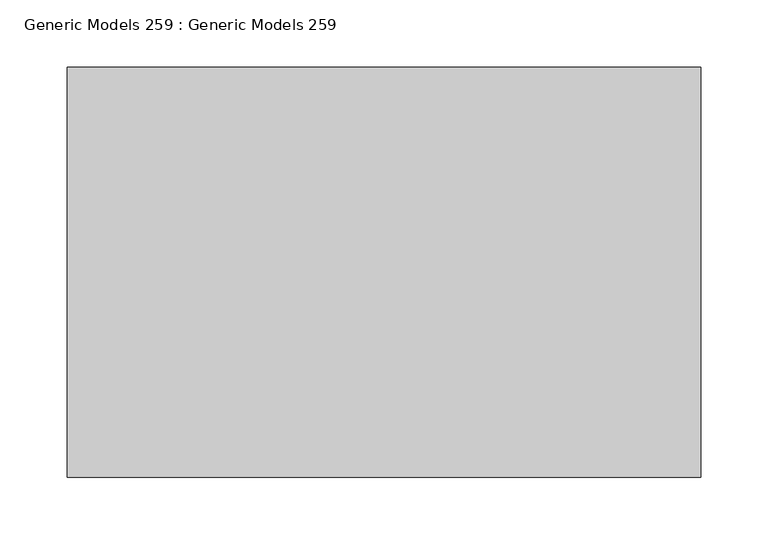
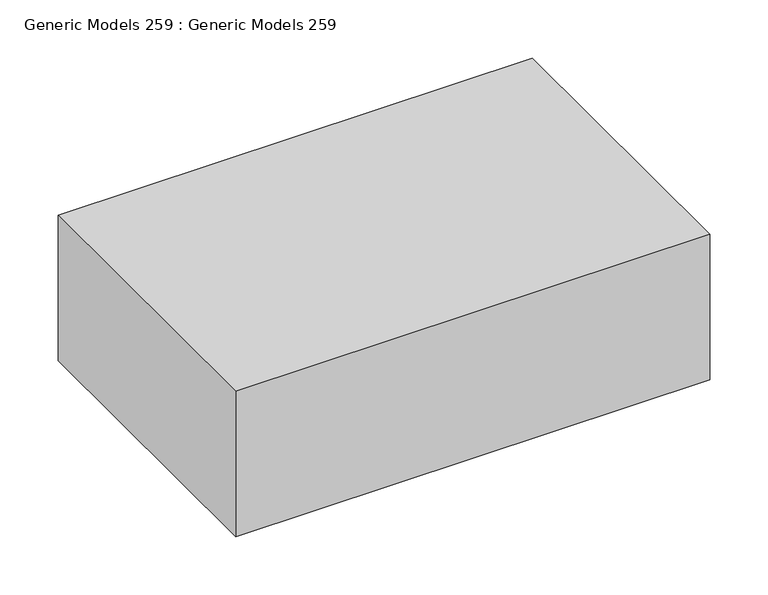
"""IFC4 building model written with IfcOpenShell, lengths in millimetres: proxy geometry, Generic Models 259 : Generic Models 259."""

import ifcopenshell
import ifcopenshell.guid

model = None  # the IFC model being written
_history = None  # IfcOwnerHistory: only IFC2X3 demands one
_inside = {}  # id of a spatial element -> (the spatial element, [elements in it])
_under = {}  # id of a project, library or spatial element -> (it, [spatial elements below it])
_declared = {}  # id of a project -> (the project, [libraries it declares])
_typed = {}  # id of a type object -> (the type object, [elements of that type])
_made_of = {}  # id of a material, layer set ... -> (it, [elements and type objects made of it])


def new_model(schema):
    """Start an empty IFC model of exactly this schema.

    Asked for "IFC4X3", IfcOpenShell would pick the latest addendum, in which some entities
    have other attributes; the version numbers below select the first issue.
    IFC2X3 requires an IfcOwnerHistory on every rooted entity: one is made here for all.
    """
    global model, _history
    if schema == "IFC4X3":
        model = ifcopenshell.file(schema_version=(4, 3, 0, 0))
    else:
        model = ifcopenshell.file(schema=schema)
    _inside.clear()
    _under.clear()
    _declared.clear()
    _typed.clear()
    _made_of.clear()
    _history = None
    if model.schema == "IFC2X3":
        org = make("IfcOrganization", Name="unknown")
        user = make(
            "IfcPersonAndOrganization",
            ThePerson=make("IfcPerson", FamilyName="unknown"),
            TheOrganization=org,
        )
        app = make(
            "IfcApplication",
            ApplicationDeveloper=org,
            Version="unknown",
            ApplicationFullName="unknown",
            ApplicationIdentifier="unknown",
        )
        _history = make(
            "IfcOwnerHistory",
            OwningUser=user,
            OwningApplication=app,
            ChangeAction="ADDED",
            CreationDate=0,
        )
    return model


def make(cls, **values):
    """One entity of the class cls with the attributes given. An attribute that is None is left unset."""
    return model.create_entity(
        cls, **{name: value for name, value in values.items() if value is not None}
    )


def rooted(cls, **values):
    """An entity with a GlobalId (a new one), such as an element, a storey or a relation."""
    return make(cls, GlobalId=ifcopenshell.guid.new(), OwnerHistory=_history, **values)


def si_unit(unit_type, name, prefix=None):
    """IfcSIUnit, for example si_unit("LENGTHUNIT", "METRE", prefix="MILLI")."""
    return make("IfcSIUnit", UnitType=unit_type, Prefix=prefix, Name=name)


def assignment(units):
    """IfcUnitAssignment: the units of a project."""
    return None if units is None else make("IfcUnitAssignment", Units=units)


def point(xyz):
    """IfcCartesianPoint."""
    return None if xyz is None else make("IfcCartesianPoint", Coordinates=xyz)


def direction(xyz):
    """IfcDirection."""
    return None if xyz is None else make("IfcDirection", DirectionRatios=xyz)


def frame(location, z_axis=None, x_axis=None):
    """IfcAxis2Placement3D, a coordinate frame: its origin and axes. An axis left out is left unset."""
    return make(
        "IfcAxis2Placement3D",
        Location=point(location),
        Axis=direction(z_axis),
        RefDirection=direction(x_axis),
    )


def origin():
    """The frame at (0, 0, 0) with its axes left unset."""
    return frame((0.0, 0.0, 0.0))


def place(relative_to, where):
    """IfcLocalPlacement: puts the frame where relative to a parent placement (None: the world)."""
    return make(
        "IfcLocalPlacement", PlacementRelTo=relative_to, RelativePlacement=where
    )


def context(
    kind, dimensions, precision=None, world=None, true_north=None, identifier=None
):
    """IfcGeometricRepresentationContext, for example the 3D "Model" context."""
    return make(
        "IfcGeometricRepresentationContext",
        ContextIdentifier=identifier,
        ContextType=kind,
        CoordinateSpaceDimension=dimensions,
        Precision=precision,
        WorldCoordinateSystem=world,
        TrueNorth=true_north,
    )


def project(units=None, contexts=None):
    """IfcProject with its units and contexts."""
    return rooted(
        "IfcProject",
        Name="project",
        RepresentationContexts=contexts,
        UnitsInContext=assignment(units),
    )


def spatial(cls, under=None, at=None, **own):
    """A site, building, storey or space (cls), placed at a placement, below another one or the project."""
    s = rooted(cls, ObjectPlacement=at, **own)
    if under is not None:
        _under.setdefault(under.id(), (under, []))[1].append(s)
    return s


def polyline(points):
    """IfcPolyline through the points."""
    return make("IfcPolyline", Points=[point(p) for p in points])


def outline(outer, holes=None, kind="AREA"):
    """IfcArbitraryClosedProfileDef: a profile drawn as a closed curve; with holes, ...WithVoids."""
    if holes is None:
        return make("IfcArbitraryClosedProfileDef", ProfileType=kind, OuterCurve=outer)
    return make(
        "IfcArbitraryProfileDefWithVoids",
        ProfileType=kind,
        OuterCurve=outer,
        InnerCurves=holes,
    )


def extrude(swept, where, along, depth):
    """IfcExtrudedAreaSolid: the profile swept, set in the frame where, extruded along a direction by depth."""
    return make(
        "IfcExtrudedAreaSolid",
        SweptArea=swept,
        Position=where,
        ExtrudedDirection=direction(along),
        Depth=depth,
    )


def shape(context_of_items, identifier, shape_type, items):
    """IfcShapeRepresentation: the items that make up one representation, for example the "Body"."""
    return make(
        "IfcShapeRepresentation",
        ContextOfItems=context_of_items,
        RepresentationIdentifier=identifier,
        RepresentationType=shape_type,
        Items=items,
    )


def source(mapping_origin, context_of_items, identifier, shape_type, items):
    """IfcRepresentationMap: a shape defined once, which mapped items show again and again."""
    return make(
        "IfcRepresentationMap",
        MappingOrigin=mapping_origin,
        MappedRepresentation=shape(context_of_items, identifier, shape_type, items),
    )


def transform(
    local_origin,
    x_axis=None,
    y_axis=None,
    z_axis=None,
    scale=None,
    scale2=None,
    scale3=None,
    uniform=True,
):
    """IfcCartesianTransformationOperator3D, or its non-uniform kind. x_axis, y_axis, z_axis: its Axis1, 2, 3."""
    if uniform:
        return make(
            "IfcCartesianTransformationOperator3D",
            Axis1=direction(x_axis),
            Axis2=direction(y_axis),
            LocalOrigin=point(local_origin),
            Scale=scale,
            Axis3=direction(z_axis),
        )
    return make(
        "IfcCartesianTransformationOperator3DnonUniform",
        Axis1=direction(x_axis),
        Axis2=direction(y_axis),
        LocalOrigin=point(local_origin),
        Scale=scale,
        Axis3=direction(z_axis),
        Scale2=scale2,
        Scale3=scale3,
    )


def mapped(mapping_source, mapping_target):
    """IfcMappedItem: shows the shape of a source again, moved by a transform."""
    return make(
        "IfcMappedItem", MappingSource=mapping_source, MappingTarget=mapping_target
    )


def made_of(thing, what):
    """Note that an element or type object is made of a material, layer set ...; save() writes the relation."""
    if what is not None:
        _made_of.setdefault(what.id(), (what, []))[1].append(thing)
    return thing


def element(
    cls,
    number,
    at=None,
    inside=None,
    cuts=None,
    type_object=None,
    material=None,
    context=None,
    identifier="Body",
    shape_type=None,
    held_by="IfcProductDefinitionShape",
    body=None,
    shapes=None,
    **own,
):
    """One element of the class cls, such as IfcWall. Its Tag is "e" and its number.

    at: its placement. inside: the storey or other place that contains it. cuts: it is an
    opening in that element (IfcRelVoidsElement). A single representation is given by context,
    identifier, shape_type and body (its items); several are given by shapes. held_by: the class
    of the entity that holds the representations. save() writes the other relations.
    """
    e = rooted(cls, Tag="e%d" % number, ObjectPlacement=at, **own)
    if body is not None:
        shapes = [shape(context, identifier, shape_type, body)]
    if shapes is not None:
        e.Representation = make(held_by, Representations=shapes)
    if inside is not None:
        _inside.setdefault(inside.id(), (inside, []))[1].append(e)
    if cuts is not None:
        rooted(
            "IfcRelVoidsElement", RelatingBuildingElement=cuts, RelatedOpeningElement=e
        )
    if type_object is not None:
        _typed.setdefault(type_object.id(), (type_object, []))[1].append(e)
    return made_of(e, material)


def aggregate(whole, parts):
    """IfcRelAggregates: a whole, such as a stair, and the parts it consists of."""
    return rooted("IfcRelAggregates", RelatingObject=whole, RelatedObjects=parts)


def save(model, path):
    """Write the relations noted so far, then the file.

    IfcRelAggregates (storeys below a building ...), IfcRelContainedInSpatialStructure (elements
    in a storey), IfcRelDefinesByType, IfcRelAssociatesMaterial and IfcRelDeclares: one each for
    every whole, place, type object, material and project.
    """
    for whole, parts in _under.values():
        aggregate(whole, parts)
    for where, things in _inside.values():
        rooted(
            "IfcRelContainedInSpatialStructure",
            RelatedElements=things,
            RelatingStructure=where,
        )
    for kind, things in _typed.values():
        rooted("IfcRelDefinesByType", RelatedObjects=things, RelatingType=kind)
    for what, things in _made_of.values():
        rooted("IfcRelAssociatesMaterial", RelatedObjects=things, RelatingMaterial=what)
    for by, libraries in _declared.values():
        rooted("IfcRelDeclares", RelatingContext=by, RelatedDefinitions=libraries)
    model.write(path)


def generic_models_259_generic_models_259_120d9b36(model_context):
    return source(origin(), model_context, "Body", "SweptSolid", [
        extrude(outline(polyline([(2095.3263704, 4564.8872686), (2566.0251699, 4564.8872686), (2566.0251699, 4260.0872686), (2095.3263704, 4260.0872686), (2095.3263704, 4564.8872686)])), frame((0.0, 0.0, 123602.496), z_axis=(0.0, 0.0, 1.0), x_axis=(1.0, 0.0, 0.0)), (0.0, 0.0, 1.0), 152.4),
    ])


if __name__ == "__main__":
    model = new_model("IFC4")
    model_context = context("Model", 3, world=origin())
    ifc_project = project(units=[si_unit("LENGTHUNIT", "METRE", prefix="MILLI")], contexts=[model_context])
    site = spatial("IfcSite", under=ifc_project)
    building = spatial("IfcBuilding", under=site)
    placement = place(None, origin())
    generic_models_259_generic_models_259_shape = generic_models_259_generic_models_259_120d9b36(model_context)
    element("IfcBuildingElementProxy", 1, Name="Generic Models 259 : Generic Models 259", ObjectType="Generic Models 259 : Generic Models 259", at=placement, inside=building, context=model_context, shape_type="MappedRepresentation", body=[
        mapped(generic_models_259_generic_models_259_shape, transform((0.0, 0.0, 0.0), x_axis=(1.0, 0.0, 0.0), y_axis=(0.0, 1.0, 0.0), z_axis=(0.0, 0.0, 1.0))),
    ])
    save(model, "model.ifc")

# Revit data of these elements
# Element 1 (IfcBuildingElementProxy, "Generic Models 259 : Generic Models 259")
#   Materials on its faces: "_CONCRETE SLAB W/ WIRE MESH (SEE STRUCT. DWGS) - SLOPE 1% AWAY FROM BUILDING"
# Materials
#   "_CONCRETE SLAB W/ WIRE MESH (SEE STRUCT. DWGS) - SLOPE 1% AWAY FROM BUILDING": class "Generic", colour RGB 191 191 191, transparency 0, Cost = 0
